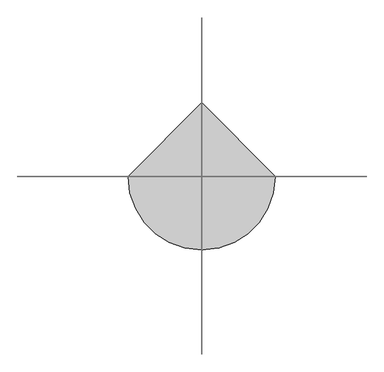
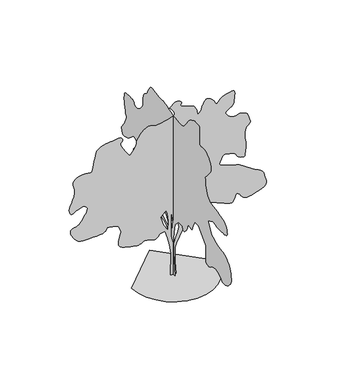
"""IFC4 building model written with IfcOpenShell, lengths in millimetres: proxy geometry, blueberry elder 26160 : blueberry elder 26160."""

from ifc_helpers import new_model, si_unit, origin, place, context, project, spatial, triangles, source, transform, mapped, element, save


def entourage_a2d70376(model_context):
    return source(origin(), model_context, "Body", "Tessellation", [
        triangles([(-0.0014919, 59.6430573, 0.0042007), (-0.0014919, -63.4980182, 0.0042007), (-0.0014919, -15.6099892, 574.662743), (-0.0014919, -1.9275415, 923.5625221), (-0.0014919, -22.4510529, 1121.9570257), (-0.0014919, -77.1804997, 1347.7149754), (-0.0014919, -227.6865383, 1498.2227943), (-0.0014919, -385.0338381, 1498.2227943), (-0.0014919, -419.2400351, 1402.4443382), (-0.0014919, -487.6499219, 1409.2870892), (-0.0014919, -562.9051031, 1498.2227943), (-0.0014919, -610.791715, 1593.9986343), (-0.0014919, -638.1577045, 1689.7744743), (-0.0014919, -713.4103786, 1662.4110283), (-0.0014919, -795.5032602, 1655.5682774), (-0.0014919, -870.7558617, 1826.5992622), (-0.0014919, -925.4852972, 1929.2153824), (-0.0014919, -1075.9931162, 1922.3751022), (-0.0014919, -1192.2921947, 1826.5992622), (-0.0014919, -1404.3696568, 1600.8387691), (-0.0014919, -1411.2099369, 1375.0808922), (-0.0014919, -1409.1144253, 1348.2534599), (-0.0014919, -1404.5093285, 1316.2824463), (-0.0014919, -1399.9017609, 1281.557967), (-0.0014919, -1397.8062492, 1246.4730446), (-0.0014919, -1400.7374657, 1213.4249891), (-0.0014919, -1411.2099369, 1184.8042797), (-0.0014919, -1431.7331028, 1163.0034302), (-0.0014919, -1457.4226685, 1147.2477785), (-0.0014919, -1482.2740585, 1135.79746), (-0.0014919, -1507.1254486, 1129.6151339), (-0.0014919, -1532.8150143, 1129.6557564), (-0.0014919, -1560.1810764, 1136.8769726), (-0.0014919, -1590.0565784, 1152.2338114), (-0.0014919, -1623.2873989, 1176.6863886), (-0.0014919, -1664.49375, 1202.6350954), (-0.0014919, -1715.0347057, 1221.7613262), (-0.0014919, -1770.8411831, 1233.9482277), (-0.0014919, -1827.8439537, 1239.0739323), (-0.0014919, -1881.9739346, 1237.0215866), (-0.0014919, -1929.1645134, 1227.6667797), (-0.0014919, -1965.3442818, 1210.8926582), (-0.0014919, -1995.2630951, 1185.7212296), (-0.0014919, -2027.0942917, 1154.4487198), (-0.0014919, -2061.9177475, 1121.8579039), (-0.0014919, -2100.8127571, 1092.7367889), (-0.0014919, -2144.8513481, 1071.8757803), (-0.0014919, -2195.1129604, 1064.0551094), (-0.0014919, -2252.6744179, 1074.0677977), (-0.0014919, -2311.551638, 1100.7352833), (-0.0014919, -2364.3279224, 1137.4535362), (-0.0014919, -2409.9209244, 1180.8748684), (-0.0014919, -2447.2590523, 1227.6464321), (-0.0014919, -2475.2625755, 1274.4181412), (-0.0014919, -2492.8519089, 1317.8368572), (-0.0014919, -2498.9556061, 1354.5577263), (-0.0014919, -2495.0465424, 1394.6871082), (-0.0014919, -2484.4370155, 1446.9019444), (-0.0014919, -2468.7981445, 1505.7005356), (-0.0014919, -2449.8115128, 1565.5759506), (-0.0014919, -2429.1486752, 1621.024165), (-0.0014919, -2408.4858376, 1666.538538), (-0.0014919, -2389.496735, 1696.6146091), (-0.0014919, -2367.4393604, 1721.5473896), (-0.0014919, -2337.0025555, 1752.8198994), (-0.0014919, -2299.0269665, 1786.7288761), (-0.0014919, -2254.3509144, 1819.5584129), (-0.0014919, -2203.8099586, 1847.6000153), (-0.0014919, -2148.2422749, 1867.1453339), (-0.0014919, -2088.4861839, 1874.4858742), (-0.0014919, -2026.3171589, 1879.471907), (-0.0014919, -1963.0710194, 1893.4344269), (-0.0014919, -1898.9284229, 1914.8745426), (-0.0014919, -1834.0668297, 1942.2988861), (-0.0014919, -1768.6668972, 1974.2114731), (-0.0014919, -1702.9062309, 2009.1161739), (-0.0014919, -1636.9678139, 2045.5143883), (-0.0014919, -1493.3027458, 2312.3213585), (-0.0014919, -1712.220488, 2414.9399494), (-0.0014919, -1741.6996479, 2406.2024014), (-0.0014919, -1772.1365982, 2397.8254417), (-0.0014919, -1804.4885479, 2390.1673336), (-0.0014919, -1839.7108166, 2383.5861946), (-0.0014919, -1878.7633747, 2378.4401424), (-0.0014919, -1922.603722, 2375.0899109), (-0.0014919, -1972.187178, 2373.8910015), (-0.0014919, -2028.8316856, 2373.6725555), (-0.0014919, -2090.261657, 2373.8122272), (-0.0014919, -2152.0522167, 2375.5064552), (-0.0014919, -2209.7738388, 2379.9564743), (-0.0014919, -2258.9965611, 2388.3511654), (-0.0014919, -2295.2982697, 2401.8945248), (-0.0014919, -2314.2440609, 2421.7802296), (-0.0014919, -2317.876252, 2453.1136368), (-0.0014919, -2312.2908371, 2496.5351143), (-0.0014919, -2299.1666382, 2546.5297371), (-0.0014919, -2280.1775356, 2597.6091774), (-0.0014919, -2257.0026421, 2644.26912), (-0.0014919, -2231.3130764, 2680.9974014), (-0.0014919, -2204.7853352, 2702.2574409), (-0.0014919, -2178.018655, 2712.9253944), (-0.0014919, -2148.9788578, 2722.1454712), (-0.0014919, -2115.3923904, 2730.9847572), (-0.0014919, -2074.9835197, 2740.5606262), (-0.0014919, -2025.478838, 2751.9398735), (-0.0014919, -1964.605228, 2766.1637146), (-0.0014919, -1890.091753, 2784.3501045), (-0.0014919, -1810.2315113, 2802.4350471), (-0.0014919, -1735.3979977, 2817.522789), (-0.0014919, -1666.4267715, 2832.4579239), (-0.0014919, -1604.1586246, 2850.1870743), (-0.0014919, -1549.4291164, 2873.5298355), (-0.0014919, -1503.0767132, 2905.3557999), (-0.0014919, -1465.9392998, 2948.5613022), (-0.0014919, -1437.478537, 3000.783696), (-0.0014919, -1415.8377068, 3057.3241402), (-0.0014919, -1399.8814133, 3117.4716316), (-0.0014919, -1388.4717899, 3180.4634262), (-0.0014919, -1380.4732956, 3245.6399712), (-0.0014919, -1374.7506798, 3312.238813), (-0.0014919, -1370.1634598, 3379.5489487), (-0.0014919, -1421.161655, 3432.3047401), (-0.0014919, -1470.3080738, 3484.9335045), (-0.0014919, -1515.7412018, 3537.3337944), (-0.0014919, -1555.6115879, 3589.3785828), (-0.0014919, -1588.0626595, 3640.9149719), (-0.0014919, -1611.2401691, 3691.8929649), (-0.0014919, -1623.2873989, 3742.1340843), (-0.0014919, -1619.2183159, 3797.684182), (-0.0014919, -1597.4378139, 3860.6506874), (-0.0014919, -1561.1766552, 3925.0397804), (-0.0014919, -1513.6685085, 3984.9076378), (-0.0014919, -1458.1415199, 4034.2345688), (-0.0014919, -1397.8265968, 4067.0258812), (-0.0014919, -1335.9572628, 4077.3383331), (-0.0014919, -1278.5939037, 4074.2649742), (-0.0014919, -1229.7292992, 4071.8773293), (-0.0014919, -1189.4804478, 4071.7755913), (-0.0014919, -1157.966601, 4075.509375), (-0.0014919, -1135.3097717, 4084.6280045), (-0.0014919, -1121.6268133, 4100.6808037), (-0.0014919, -1117.0395206, 4125.2426765), (-0.0014919, -1118.7743711, 4171.0390091), (-0.0014919, -1122.5437632, 4241.9559013), (-0.0014919, -1126.1936857, 4326.2838936), (-0.0014919, -1127.5704185, 4412.288237), (-0.0014919, -1124.5173346, 4488.2344734), (-0.0014919, -1114.885655, 4542.4125618), (-0.0014919, -1096.5163548, 4563.0627548), (-0.0014919, -1069.6304232, 4564.4597626), (-0.0014919, -1037.2377783, 4567.5331215), (-0.0014919, -1001.3780485, 4570.6067711), (-0.0014919, -964.0806158, 4572.0037788), (-0.0014919, -927.380167, 4570.0477936), (-0.0014919, -893.3136417, 4563.0627548), (-0.0014919, -863.9156542, 4549.3976006), (-0.0014919, -835.993376, 4533.1416161), (-0.0014919, -805.556571, 4518.3587975), (-0.0014919, -773.4433422, 4503.0678703), (-0.0014919, -740.4944086, 4485.3895889), (-0.0014919, -707.545475, 4463.4185463), (-0.0014919, -675.4347897, 4435.2246277), (-0.0014919, -644.9979847, 4398.877137), (-0.0014919, -614.4824055, 4355.0112099), (-0.0014919, -581.8128516, 4307.6911331), (-0.0014919, -547.3475862, 4260.1167114), (-0.0014919, -511.4446541, 4215.5397812), (-0.0014919, -474.4672963, 4177.1857269), (-0.0014919, -436.7711234, 4148.2805145), (-0.0014919, -398.7168328, 4132.075399), (-0.0014919, -359.7633602, 4126.0048393), (-0.0014919, -319.1360072, 4124.6078316), (-0.0014919, -276.8322849, 4126.6905533), (-0.0014919, -232.8521387, 4131.0338928), (-0.0014919, -187.1978941, 4136.4696075), (-0.0014919, -139.8680069, 4141.7780045), (-0.0014919, -90.8629858, 4145.7658424), (-0.0014919, -33.0220578, 4153.2081207), (-0.0014919, 35.9481419, 4167.7368851), (-0.0014919, 108.7479043, 4186.3296455), (-0.0014919, 178.0769938, 4205.989492), (-0.0014919, 236.6359921, 4223.7439316), (-0.0014919, 277.1243819, 4236.5963448), (-0.0014919, 292.2424816, 4241.523951), (-0.0014919, 300.5609782, 4244.1147812), (-0.0014919, 323.5962728, 4250.5411331), (-0.0014919, 358.4806623, 4258.7705727), (-0.0014919, 402.3388501, 4266.7462486), (-0.0014919, 452.3032422, 4272.4357269), (-0.0014919, 505.495962, 4273.8327347), (-0.0014919, 559.0493792, 4268.9051285), (-0.0014919, 618.0663437, 4267.9400711), (-0.0014919, 686.0596498, 4278.836499), (-0.0014919, 757.7613779, 4295.8293571), (-0.0014919, 827.9085497, 4313.1774261), (-0.0014919, 891.2359343, 4325.1409401), (-0.0014919, 942.4728504, 4325.9789703), (-0.0014919, 976.3615522, 4309.9517509), (-0.0014919, 999.7371603, 4282.3926773), (-0.0014919, 1022.6327831, 4252.7761711), (-0.0014919, 1044.5733044, 4221.6359207), (-0.0014919, 1065.0761953, 4189.4032951), (-0.0014919, 1083.6639416, 4156.5608231), (-0.0014919, 1099.8614994, 4123.6171944), (-0.0014919, 1113.1837967, 4091.0287766), (-0.0014919, 1129.0994677, 4063.2159393), (-0.0014919, 1151.7182178, 4042.0067688), (-0.0014919, 1178.5228317, 4023.896537), (-0.0014919, 1207.0064129, 4005.4308037), (-0.0014919, 1234.6492023, 3983.1295486), (-0.0014919, 1258.9419056, 3953.5130424), (-0.0014919, 1277.3720306, 3913.1524246), (-0.0014919, 1288.5608826, 3878.2275215), (-0.0014919, 1294.0066257, 3861.6157448), (-0.0014919, 1295.50261, 3854.8086021), (-0.0014919, 1294.8448013, 3849.3223091), (-0.0014919, 1293.8262589, 3836.6730812), (-0.0014919, 1294.245274, 3808.3265556), (-0.0014919, 1297.8953419, 3755.7995293), (-0.0014919, 1304.3392799, 3695.8046448), (-0.0014919, 1312.5765678, 3648.6365936), (-0.0014919, 1323.5645599, 3611.1208603), (-0.0014919, 1338.2635174, 3580.2090843), (-0.0014919, 1357.6310852, 3552.7770378), (-0.0014919, 1382.622147, 3525.6752037), (-0.0014919, 1414.1969639, 3495.8555122), (-0.0014919, 1450.0566936, 3466.1628479), (-0.0014919, 1486.6377457, 3441.8806091), (-0.0014919, 1522.9750626, 3423.3131378), (-0.0014919, 1558.118557, 3410.8670952), (-0.0014919, 1591.1081131, 3404.8979828), (-0.0014919, 1620.9860859, 3405.7363037), (-0.0014919, 1646.795121, 3413.7628487), (-0.0014919, 1665.9440975, 3429.5107246), (-0.0014919, 1679.3451691, 3450.9992386), (-0.0014919, 1691.3136246, 3474.7736595), (-0.0014919, 1706.1523991, 3497.354258), (-0.0014919, 1728.1716946, 3515.2613045), (-0.0014919, 1761.6793877, 3525.0403587), (-0.0014919, 1810.9833549, 3523.2114006), (-0.0014919, 1870.0002468, 3519.655513), (-0.0014919, 1927.9427856, 3522.4495285), (-0.0014919, 1982.0524189, 3525.3702805), (-0.0014919, 2029.5835293, 3522.1698944), (-0.0014919, 2067.7775642, 3506.6504929), (-0.0014919, 2093.8862904, 3472.5891998), (-0.0014919, 2105.1536259, 3413.7628487), (-0.0014919, 2107.5870529, 3355.0888138), (-0.0014919, 2108.7045719, 3318.9189285), (-0.0014919, 2108.0264156, 3295.0939293), (-0.0014919, 2105.0749969, 3273.4275192), (-0.0014919, 2099.3701126, 3243.7095657), (-0.0014919, 2090.4343208, 3195.8305115), (-0.0014919, 2077.7901798, 3119.5796425), (-0.0014919, 2061.2548519, 3041.6777115), (-0.0014919, 2043.5255562, 2988.8966309), (-0.0014919, 2028.4253151, 2951.2030014), (-0.0014919, 2019.7893597, 2918.5384254), (-0.0014919, 2021.4453632, 2880.844796), (-0.0014919, 2037.2212898, 2828.0637154), (-0.0014919, 2070.9474289, 2750.1617844), (-0.0014919, 2114.4501514, 2668.4752007), (-0.0014919, 2155.0774681, 2607.7440239), (-0.0014919, 2189.9618214, 2562.9383286), (-0.0014919, 2216.2279507, 2529.0063881), (-0.0014919, 2231.0082985, 2500.9418221), (-0.0014919, 2231.4273136, 2473.7181931), (-0.0014919, 2214.6124969, 2442.3032501), (-0.0014919, 2195.0062809, 2409.7735497), (-0.0014919, 2184.256937, 2383.1061367), (-0.0014919, 2175.300943, 2363.1416576), (-0.0014919, 2161.0794273, 2350.7159626), (-0.0014919, 2134.5339546, 2346.6672272), (-0.0014919, 2088.6004211, 2351.8336269), (-0.0014919, 2016.218066, 2367.0507214), (-0.0014919, 1937.2366951, 2396.3496597), (-0.0014919, 1873.5715405, 2438.0946407), (-0.0014919, 1821.2754593, 2484.6274109), (-0.0014919, 1776.3986927, 2528.2875366), (-0.0014919, 1734.9940979, 2561.4142937), (-0.0014919, 1693.1069744, 2576.3494286), (-0.0014919, 1646.795121, 2565.45271), (-0.0014919, 1602.1392712, 2539.6566101), (-0.0014919, 1566.8155552, 2514.9450371), (-0.0014919, 1539.2717422, 2491.129921), (-0.0014919, 1517.9509506, 2468.0336563), (-0.0014919, 1501.2961533, 2445.4757309), (-0.0014919, 1487.7527939, 2423.2762138), (-0.0014919, 1475.7666069, 2401.2569183), (-0.0014919, 1494.8139908, 2382.2881634), (-0.0014919, 1513.8006226, 2363.8605091), (-0.0014919, 1532.6702557, 2346.5072079), (-0.0014919, 1551.3570511, 2330.7719765), (-0.0014919, 1569.8076691, 2317.1879219), (-0.0014919, 1587.9584507, 2306.2990517), (-0.0014919, 1605.7486439, 2298.6383274), (-0.0014919, 1624.7173988, 2295.1686264), (-0.0014919, 1645.2405647, 2294.3304508), (-0.0014919, 1665.5250824, 2292.895364), (-0.0014919, 1683.7749859, 2287.6299877), (-0.0014919, 1698.1945999, 2275.3032692), (-0.0014919, 1706.9905746, 2252.6845917), (-0.0014919, 1708.3672348, 2216.5455185), (-0.0014919, 1703.8180939, 2176.2559719), (-0.0014919, 1696.2794552, 2141.3512711), (-0.0014919, 1686.106675, 2108.8417728), (-0.0014919, 1673.6606323, 2075.7328926), (-0.0014919, 1659.3020611, 2039.0323711), (-0.0014919, 1643.3838467, 1995.7533268), (-0.0014919, 1626.2718098, 1942.8984135), (-0.0014919, 1608.601086, 1883.4013184), (-0.0014919, 1592.1266556, 1823.7848991), (-0.0014919, 1578.8829872, 1766.4443584), (-0.0014919, 1570.9048405, 1713.7673412), (-0.0014919, 1570.2266842, 1668.1539917), (-0.0014919, 1578.8829872, 1631.9944256), (-0.0014919, 1598.9083637, 1607.6815201), (-0.0014919, 1624.6970512, 1591.4839622), (-0.0014919, 1649.4087696, 1577.8035473), (-0.0014919, 1673.2237404, 1566.2135571), (-0.0014919, 1696.320005, 1556.3023888), (-0.0014919, 1718.8777851, 1547.6460857), (-0.0014919, 1741.0774475, 1539.8279583), (-0.0014919, 1763.096743, 1532.4263752), (-0.0014919, 1786.3707584, 1542.3400143), (-0.0014919, 1808.5702755, 1550.1581417), (-0.0014919, 1828.6159996, 1553.787862), (-0.0014919, 1845.4283455, 1551.135989), (-0.0014919, 1857.9352856, 1540.1073017), (-0.0014919, 1865.0549091, 1518.6062885), (-0.0014919, 1865.7127178, 1484.5397633), (-0.0014919, 1859.7895329, 1448.2787498), (-0.0014919, 1848.4813568, 1420.635815), (-0.0014919, 1832.6850826, 1400.1710758), (-0.0014919, 1813.2973125, 1385.4517708), (-0.0014919, 1791.2171196, 1375.040197), (-0.0014919, 1767.3435768, 1367.5015583), (-0.0014919, 1742.570961, 1361.3978611), (-0.0014919, 1730.8234222, 1353.9581989), (-0.0014919, 1718.9565594, 1345.8607281), (-0.0014919, 1706.8509029, 1336.4474945), (-0.0014919, 1694.3845127, 1325.0580734), (-0.0014919, 1681.4406807, 1311.0372723), (-0.0014919, 1667.8974667, 1293.7246662), (-0.0014919, 1653.6378719, 1272.4623013), (-0.0014919, 1633.9909607, 1249.8053993), (-0.0014919, 1605.3701786, 1228.5837296), (-0.0014919, 1569.2691845, 1208.558353), (-0.0014919, 1527.1838173, 1189.4905489), (-0.0014919, 1480.6129681, 1171.1415962), (-0.0014919, 1431.0498596, 1153.270158), (-0.0014919, 1379.9907669, 1135.6399841), (-0.0014919, 1215.8024603, 1231.4158241), (-0.0014919, 1051.6141537, 1108.2739946), (-0.0014919, 1029.6533575, 1105.4215525), (-0.0014919, 1007.8727829, 1103.0492409), (-0.0014919, 986.4529421, 1101.6318855), (-0.0014919, 965.5690424, 1101.6522331), (-0.0014919, 945.4065376, 1103.5877254), (-0.0014919, 926.1380917, 1107.915877), (-0.0014919, 907.9491583, 1115.1167456), (-0.0014919, 891.075915, 1124.6493759), (-0.0014919, 875.1577005, 1135.2589754), (-0.0014919, 859.4808231, 1146.3486328), (-0.0014919, 843.3263586, 1157.3188934), (-0.0014919, 825.97313, 1167.5703753), (-0.0014919, 806.7071548, 1176.5060944), (-0.0014919, 784.8072561, 1183.5266687), (-0.0014919, 760.1565805, 1188.9927595), (-0.0014919, 733.3493505, 1193.7399988), (-0.0014919, 704.7489887, 1197.8877834), (-0.0014919, 674.710924, 1201.5581263), (-0.0014919, 643.59589, 1204.8677353), (-0.0014919, 611.7645481, 1207.9411669), (-0.0014919, 579.5725814, 1210.8926582), (-0.0014919, 367.4951194, 1149.3204718), (-0.0014919, 189.6253804, 1019.3383621), (-0.0014919, 93.8490136, 861.9928791), (-0.0014919, 45.9605758, 560.9797846), (-0.0013978, 66.484046, 1115.1167456), (-0.0013978, 169.1019057, 1334.0344151), (-0.0013978, 4.9135321, 1402.4443382), (-0.0014104, 312.7656838, 1190.3694197), (-0.0014104, 476.9539541, 1299.8282181), (-0.0014104, 606.9360274, 1306.6684982), (-0.0014104, 716.3948622, 1368.2381413), (-0.0014104, 710.4918795, 1371.410622), (-0.0014104, 704.3476324, 1376.0181896), (-0.0014104, 697.7284143, 1383.4984016), (-0.0014104, 690.3878014, 1395.2840195), (-0.0014104, 682.089616, 1412.8176876), (-0.0014104, 672.5976082, 1437.529406), (-0.0014104, 661.6654266, 1470.8567322), (-0.0014104, 652.9303493, 1503.7853909), (-0.0014104, 649.5801178, 1527.3819157), (-0.0014104, 650.7155136, 1543.1985374), (-0.0014104, 655.442478, 1552.7921379), (-0.0014104, 662.864336, 1557.7172733), (-0.0014104, 672.0769278, 1559.5332962), (-0.0014104, 682.1912086, 1559.7924374), (-0.0014104, 689.0314161, 1641.8852463), (-0.0014104, 606.9360274, 1696.6146091), (-0.0014104, 429.0673059, 1546.1094063), (-0.0014104, 305.9254764, 1402.4443382), (-0.0014104, 223.8310687, 1286.1453323), (-0.0014104, 141.7369426, 1101.4337872), (67.7022311, 0.0002671, 0.0), (-69.1215849, 0.0002671, 0.0), (-62.2805962, 0.0002309, 560.9772411), (-96.4865524, 0.0002173, 807.2583567), (-144.3744815, 0.0002037, 1012.4930677), (-205.9448967, 0.0001946, 1197.2045403), (-329.0852182, 0.0001946, 1183.5241253), (-349.6693906, 0.0001946, 1154.5020596), (-370.6116806, 0.0001992, 1127.2782852), (-392.2728221, 0.0001992, 1103.6436087), (-415.0109327, 0.0001992, 1085.3936325), (-439.1841302, 0.0002037, 1074.3243227), (-465.1505685, 0.0002037, 1072.2288111), (-493.2734885, 0.0001992, 1080.9054617), (-523.1921565, 0.0001992, 1093.9686905), (-554.1877936, 0.0001992, 1104.1617456), (-586.0800694, 0.0001992, 1111.9595255), (-618.6886168, 0.0001992, 1117.8447041), (-651.8381922, 0.0001992, 1122.2922523), (-685.3458853, 0.0001992, 1125.7822283), (-719.0339453, 0.0001992, 1128.7946898), (-746.9764984, 0.0001992, 1112.8383963), (-775.4575361, 0.0001992, 1097.8981018), (-805.0180864, 0.0001992, 1084.9948923), (-836.191547, 0.0001992, 1075.1422234), (-869.5188732, 0.0002037, 1069.3586374), (-905.5412384, 0.0002037, 1068.6601336), (-944.7918222, 0.0002037, 1074.0652542), (-995.5334925, 0.0001992, 1083.856953), (-1060.8724548, 0.0001992, 1096.2826481), (-1133.6334206, 0.0001992, 1112.2999117), (-1206.6330345, 0.0001992, 1132.8637728), (-1272.690921, 0.0001946, 1158.9318037), (-1324.6262684, 0.0001946, 1191.4615768), (-1355.2613171, 0.0001901, 1231.4107372), (-1365.1546085, 0.0001901, 1279.0206219), (-1362.3630638, 0.0001856, 1331.6544731), (-1350.9534405, 0.0001811, 1385.9672916), (-1334.997147, 0.0001811, 1438.6012882), (-1318.5632664, 0.0001765, 1486.2110275), (-1305.7185562, 0.0001765, 1525.4413364), (-1300.5318089, 0.000172, 1552.9470703), (-1302.9068092, 0.000172, 1576.4623501), (-1309.4676006, 0.000172, 1604.5243), (-1319.3812397, 0.0001675, 1634.9815979), (-1331.8069347, 0.0001675, 1665.6773987), (-1345.9089809, 0.000163, 1694.4582001), (-1360.8467319, 0.000163, 1719.1699184), (-1375.7869537, 0.000163, 1737.6586155), (-1395.4313942, 0.000163, 1750.9224861), (-1424.0546471, 0.0001584, 1761.6716846), (-1460.1531704, 0.0001584, 1770.328133), (-1502.2385376, 0.0001584, 1777.3079395), (-1548.8093868, 0.0001584, 1783.0331715), (-1598.3724953, 0.0001584, 1787.9200825), (-1649.431588, 0.0001584, 1792.3879784), (-1657.3716557, 0.0001584, 1766.1802757), (-1668.9591751, 0.000163, 1741.0495422), (-1687.8465397, 0.000163, 1718.0726017), (-1717.6865788, 0.000163, 1698.3265686), (-1762.1238373, 0.000163, 1682.8885574), (-1824.8111446, 0.0001675, 1672.8377174), (-1909.398278, 0.0001675, 1669.2462215), (-2003.1193016, 0.0001675, 1666.9119164), (-2090.3809811, 0.0001675, 1662.3043488), (-2170.5789928, 0.0001675, 1659.0150146), (-2243.1190418, 0.0001675, 1660.6304684), (-2307.4039261, 0.0001675, 1670.7422058), (-2362.8293221, 0.000163, 1692.9418682), (-2408.80326, 0.000163, 1730.8183353), (-2450.3908379, 0.0001584, 1780.5998898), (-2490.1799789, 0.0001584, 1834.2117336), (-2523.8680389, 0.0001539, 1888.783548), (-2547.1392929, 0.0001494, 1941.4378922), (-2555.6992355, 0.0001449, 1989.3067726), (-2545.2344673, 0.0001449, 2029.5149288), (-2511.4219963, 0.0001449, 2059.1923325), (-2467.3223625, 0.0001403, 2077.8410488), (-2428.3689262, 0.0001403, 2089.431039), (-2393.8453068, 0.0001403, 2097.7876511), (-2363.0298912, 0.0001403, 2106.7437904), (-2335.2067348, 0.0001403, 2120.1269852), (-2309.6568409, 0.0001358, 2141.7653446), (-2285.6615032, 0.0001358, 2175.4939545), (-2257.2616379, 0.0001313, 2219.9110107), (-2222.6364258, 0.0001313, 2269.4739738), (-2187.2922169, 0.0001267, 2321.7904026), (-2156.7360878, 0.0001222, 2374.464949), (-2136.4719177, 0.0001222, 2425.1076427), (-2132.0040218, 0.0001177, 2471.3203743), (-2148.8391861, 0.0001177, 2510.7107025), (-2179.7535782, 0.0001132, 2538.5136566), (-2213.5406147, 0.0001132, 2553.0322472), (-2249.7203831, 0.0001132, 2556.4866875), (-2287.8154415, 0.0001132, 2551.0765526), (-2327.3479122, 0.0001132, 2539.0342644), (-2367.8355572, 0.0001132, 2522.5573631), (-2408.80326, 0.0001177, 2503.8704224), (-2437.9625267, 0.0001177, 2487.9929031), (-2466.1666191, 0.0001177, 2473.6141296), (-2492.453096, 0.0001177, 2462.2247086), (-2515.8670738, 0.0001177, 2455.3233856), (-2535.4554131, 0.0001177, 2454.4065811), (-2550.2635208, 0.0001177, 2460.9672272), (-2559.3059921, 0.0001177, 2476.5046509), (-2566.1387146, 0.0001177, 2495.7526039), (-2573.6824402, 0.0001177, 2514.0433479), (-2580.1340813, 0.0001132, 2533.7688881), (-2583.7155487, 0.0001132, 2557.3247177), (-2582.6487534, 0.0001132, 2587.0935402), (-2575.1047371, 0.0001086, 2625.4984634), (-2559.3059921, 0.0001041, 2674.9015526), (-2538.1680382, 0.0001041, 2727.6064751), (-2516.667025, 9.96e-05, 2775.7904526), (-2496.1235115, 9.96e-05, 2821.5612053), (-2477.8534058, 9.51e-05, 2867.0781944), (-2463.1746506, 9.05e-05, 2914.5505875), (-2453.4005379, 9.05e-05, 2966.0619781), (-2449.8498825, 8.6e-05, 3023.7962448), (-2453.8603935, 8.15e-05, 3079.1681557), (-2463.4920731, 8.15e-05, 3124.1261673), (-2475.1608376, 7.7e-05, 3161.6674805), (-2485.2727203, 7.7e-05, 3194.7637161), (-2490.240731, 7.24e-05, 3226.4376549), (-2486.4688683, 7.24e-05, 3259.6609177), (-2470.3753738, 6.79e-05, 3297.4559944), (-2440.0783859, 6.79e-05, 3333.6511688), (-2398.8922371, 6.34e-05, 3360.8800301), (-2351.003009, 6.34e-05, 3380.2093735), (-2300.601725, 6.34e-05, 3392.7059944), (-2251.8769375, 6.34e-05, 3399.4625587), (-2209.0144375, 6.34e-05, 3401.5708603), (-2176.2051029, 6.34e-05, 3400.0721146), (-2148.061908, 6.34e-05, 3394.4587944), (-2117.7647747, 6.34e-05, 3386.2290642), (-2087.3483173, 6.34e-05, 3379.4219215), (-2058.8468594, 6.34e-05, 3378.1263611), (-2034.2926895, 6.34e-05, 3386.4069603), (-2015.7253635, 6.34e-05, 3408.3271339), (-2005.174118, 5.88e-05, 3447.9511688), (-1996.2586739, 5.43e-05, 3505.228196), (-1982.4359711, 5.43e-05, 3573.6559959), (-1965.5043011, 4.98e-05, 3647.5697983), (-1947.2543976, 4.53e-05, 3721.3568642), (-1929.4820812, 4.07e-05, 3789.4035828), (-1913.985498, 3.62e-05, 3846.0963432), (-1902.5555271, 3.17e-05, 3885.7968269), (-1882.1516853, 3.17e-05, 3914.5241432), (-1842.3625443, 3.17e-05, 3941.473661), (-1788.9284512, 2.72e-05, 3965.6797417), (-1727.5976017, 2.72e-05, 3986.1523293), (-1664.1128139, 2.72e-05, 4001.9763634), (-1604.2170513, 2.72e-05, 4012.1617882), (-1553.655748, 2.72e-05, 4015.7685448), (-1506.505719, 2.72e-05, 4019.2738541), (-1455.4059311, 2.72e-05, 4027.0969231), (-1403.9480255, 2.72e-05, 4035.1487572), (-1355.7210274, 2.26e-05, 4039.3906494), (-1314.3139618, 2.72e-05, 4035.7077347), (-1283.3207954, 2.72e-05, 4020.0865952), (-1266.3256119, 2.72e-05, 3988.4126564), (-1265.9090675, 3.17e-05, 3953.5130424), (-1277.2170982, 3.17e-05, 3927.1225021), (-1292.7136814, 3.17e-05, 3903.5003975), (-1304.8625038, 3.62e-05, 3876.8813828), (-1306.1173691, 3.62e-05, 3841.4989494), (-1288.9442894, 4.07e-05, 3791.6642006), (-1245.8049168, 4.53e-05, 3721.6109184), (-1194.5655298, 4.98e-05, 3646.731768), (-1155.891437, 4.98e-05, 3586.6860146), (-1126.4324793, 5.43e-05, 3542.0835045), (-1102.8384253, 5.43e-05, 3513.5340843), (-1081.7563545, 5.88e-05, 3501.5958595), (-1059.8361809, 5.43e-05, 3506.9045471), (-1033.7274548, 5.43e-05, 3530.0441231), (-1006.0846653, 5.43e-05, 3563.4705711), (-981.7894913, 4.98e-05, 3598.9288719), (-960.8472376, 4.98e-05, 3635.9620766), (-943.2576862, 4.53e-05, 3674.0620766), (-929.0158957, 4.53e-05, 3712.7463432), (-918.1268801, 4.07e-05, 3751.557637), (-910.5856253, 4.07e-05, 3790.0131386), (-896.7832701, 3.62e-05, 3834.3363052), (-868.8610645, 3.17e-05, 3887.3714401), (-829.4503887, 3.17e-05, 3943.65783), (-781.1826954, 2.72e-05, 3997.6838928), (-726.6920534, 2.26e-05, 4043.9118851), (-668.6123863, 2.26e-05, 4076.8558044), (-609.5750742, 2.26e-05, 4091.0287766), (-561.6655712, 2.26e-05, 4089.1745293), (-529.5548495, 2.26e-05, 4080.3608231), (-504.7415749, 2.26e-05, 4068.5752052), (-478.734514, 2.26e-05, 4057.7549355), (-443.0322238, 2.26e-05, 4051.836692), (-389.1410002, 2.26e-05, 4054.7577347), (-308.5619797, 2.26e-05, 4070.5056107), (-218.1912603, 2.26e-05, 4091.0034874), (-140.9838273, 2.26e-05, 4107.2086029), (-77.5383903, 1.81e-05, 4121.4836037), (-28.4536116, 1.81e-05, 4136.2408424), (5.6723577, 1.81e-05, 4153.8685455), (24.2412211, 1.81e-05, 4176.7540672), (26.6545277, 1.36e-05, 4207.310051), (18.5968788, 1.36e-05, 4240.5080246), (6.5899843, 9.1e-06, 4270.098951), (-8.707838, 9.1e-06, 4296.7182564), (-26.6385244, 9.1e-06, 4320.924337), (-46.5435071, 4.5e-06, 4343.3526192), (-67.764968, 4.5e-06, 4364.5617897), (-89.6448007, 4.5e-06, 4385.1864029), (-61.8612404, 4.5e-06, 4411.3740486), (-34.4965295, 0.0, 4436.3675812), (-7.9696625, 0.0, 4458.9734688), (17.3007665, 0.0, 4477.9728905), (40.8958095, 0.0, 4492.1967316), (62.3966728, -4.5e-06, 4500.4264618), (81.3844583, -4.5e-06, 4501.4932571), (101.1299282, -4.5e-06, 4497.6833153), (123.747879, 0.0, 4491.9682571), (147.0833914, 0.0, 4484.0687393), (168.9832901, 0.0, 4473.8071564), (187.292892, 0.0, 4460.9038742), (199.8582769, 0.0, 4445.1304184), (204.5255429, 0.0, 4426.2330254), (200.2771285, 4.5e-06, 4409.087851), (190.6436686, 4.5e-06, 4397.0737587), (180.2923927, 4.5e-06, 4387.8281021), (173.8900582, 4.5e-06, 4378.9382378), (176.103931, 4.5e-06, 4367.9906502), (191.6012409, 4.5e-06, 4352.6491447), (225.0492538, 9.1e-06, 4330.4749168), (270.045399, 9.1e-06, 4307.8943184), (316.1184952, 9.1e-06, 4291.4095688), (361.8334373, 9.1e-06, 4278.7603409), (405.7526316, 9.1e-06, 4267.6860168), (446.4409184, 1.36e-05, 4255.8751099), (482.4607038, 1.36e-05, 4241.0667114), (512.3793717, 1.36e-05, 4221.0007851), (536.1741039, 1.36e-05, 4195.1436424), (555.3003347, 1.81e-05, 4164.9937386), (570.5378131, 1.81e-05, 4131.2623672), (582.6637808, 2.26e-05, 4094.6355331), (592.4580231, 2.26e-05, 4055.8498192), (600.6952383, 2.72e-05, 4015.6415176), (608.1552117, 2.72e-05, 3974.722213), (703.9310881, 2.26e-05, 4063.647599), (703.2935543, 2.26e-05, 4067.2543556), (702.1759626, 2.26e-05, 4077.3127533), (701.7771498, 2.26e-05, 4092.7307076), (703.2935543, 2.26e-05, 4112.4920013), (707.9213968, 1.81e-05, 4135.4533905), (716.8571886, 1.81e-05, 4160.59953), (731.2970776, 1.81e-05, 4186.7868851), (747.8502823, 1.36e-05, 4214.0666153), (763.2096645, 1.36e-05, 4241.5748199), (778.6859001, 9.1e-06, 4267.025592), (795.599766, 9.1e-06, 4288.2091827), (815.2644814, 9.1e-06, 4302.7888161), (838.9982071, 9.1e-06, 4308.5038742), (868.119322, 9.1e-06, 4303.0937393), (898.3758327, 9.1e-06, 4289.9872719), (925.0433184, 9.1e-06, 4274.3408432), (948.7186901, 1.36e-05, 4256.6116928), (969.9988592, 1.36e-05, 4237.2059006), (989.4857512, 1.36e-05, 4216.5304184), (1007.7737337, 1.36e-05, 4195.0419044), (1025.4674212, 1.81e-05, 4173.1217308), (1029.993671, 1.81e-05, 4151.4047424), (1035.2997425, 1.81e-05, 4131.2879471), (1042.1602976, 1.81e-05, 4114.4224068), (1051.3550852, 2.26e-05, 4102.3827347), (1063.6613834, 2.26e-05, 4096.8199928), (1079.8564705, 2.26e-05, 4099.3346649), (1100.7200226, 2.26e-05, 4111.5522331), (1123.5978413, 1.81e-05, 4132.811982), (1146.3537197, 1.81e-05, 4159.3295494), (1170.5472284, 1.81e-05, 4188.0062874), (1197.732851, 1.36e-05, 4215.7429665), (1229.4650711, 1.36e-05, 4239.3903603), (1267.3009884, 1.36e-05, 4255.8751099), (1312.7950138, 1.36e-05, 4262.0471169), (1361.8805351, 9.1e-06, 4267.2796463), (1408.0932667, 9.1e-06, 4278.7350517), (1449.398885, 9.1e-06, 4290.06343), (1483.7651012, 9.1e-06, 4294.9148781), (1509.1549759, 9.1e-06, 4286.9900711), (1523.5363655, 1.36e-05, 4259.888237), (1524.8724758, 1.36e-05, 4207.310051), (1519.9652172, 1.81e-05, 4142.8703796), (1515.7766647, 2.26e-05, 4084.5009773), (1510.5112885, 2.72e-05, 4032.4817688), (1502.3755932, 2.72e-05, 3987.0412285), (1489.5689621, 3.17e-05, 3948.43312), (1470.3029869, 3.17e-05, 3916.8862083), (1442.7795216, 3.17e-05, 3892.6292587), (1408.3320602, 3.62e-05, 3872.7156487), (1372.4519829, 3.62e-05, 3853.18312), (1339.5615486, 3.62e-05, 3832.6852432), (1314.0928997, 3.62e-05, 3809.9014595), (1300.4709114, 4.07e-05, 3783.5362083), (1303.1226391, 4.07e-05, 3752.243351), (1326.4778996, 4.53e-05, 3714.7529068), (1361.2023788, 4.53e-05, 3678.8882355), (1394.8497437, 4.98e-05, 3652.3703773), (1427.1814911, 4.98e-05, 3633.6253006), (1457.9560661, 4.98e-05, 3621.1030998), (1486.937582, 4.98e-05, 3613.2291618), (1513.8818676, 4.98e-05, 3608.4791611), (1538.5553616, 4.98e-05, 3605.3043549), (1559.4774857, 4.98e-05, 3606.8028099), (1576.9297634, 4.98e-05, 3614.7531967), (1593.3026012, 4.98e-05, 3625.5734665), (1610.9962887, 4.98e-05, 3635.7080223), (1632.3958546, 4.98e-05, 3641.4992386), (1659.9014431, 4.98e-05, 3639.4165169), (1695.9009899, 4.98e-05, 3625.8275208), (1734.0771481, 4.98e-05, 3609.6729836), (1766.7466656, 4.98e-05, 3599.6145859), (1794.2701309, 4.98e-05, 3591.7153587), (1817.0082779, 4.98e-05, 3582.0124626), (1835.316608, 5.43e-05, 3566.5945084), (1849.558326, 5.43e-05, 3541.4486595), (1860.0892239, 5.88e-05, 3502.6882347), (1872.6545906, 5.88e-05, 3459.6350487), (1889.4085098, 6.34e-05, 3423.0590836), (1905.3241081, 6.34e-05, 3391.0296432), (1915.3774189, 6.34e-05, 3361.6419022), (1914.5392433, 6.79e-05, 3332.939875), (1897.7853241, 6.79e-05, 3303.0693146), (1860.0892239, 7.24e-05, 3270.0748169), (1819.3424377, 7.24e-05, 3225.0150673), (1794.6308647, 7.7e-05, 3164.2835999), (1782.7233067, 8.15e-05, 3093.9765541), (1780.3890015, 8.6e-05, 3020.2147774), (1784.397187, 9.05e-05, 2949.0694107), (1791.5192814, 9.51e-05, 2886.6615921), (1798.5195808, 9.51e-05, 2839.0871704), (1802.5886639, 9.96e-05, 2800.3776146), (1803.4268394, 9.96e-05, 2760.5756836), (1801.5701214, 0.0001041, 2719.8848534), (1797.5619358, 0.0001041, 2678.48302), (1791.9384418, 0.0001086, 2636.5474983), (1785.2353626, 0.0001086, 2594.2311859), (1777.9964149, 0.0001132, 2551.7622665), (1779.0935863, 0.0001132, 2530.0377205), (1777.9760674, 0.0001177, 2509.9334244), (1772.4312023, 0.0001177, 2493.0603264), (1760.2443008, 0.0001177, 2481.0334442), (1739.2028526, 0.0001177, 2475.4680862), (1707.0896965, 0.0001177, 2477.9801422), (1661.6947929, 0.0001177, 2490.1875366), (1618.3547058, 0.0001177, 2511.8867935), (1589.7339237, 0.0001132, 2539.8115425), (1569.6094254, 0.0001132, 2570.9645828), (1551.7583347, 0.0001086, 2602.3591782), (1529.9574852, 0.0001086, 2631.0103363), (1497.9864716, 0.0001086, 2653.895858), (1449.6198017, 0.0001086, 2668.0688301), (1395.7870411, 0.0001041, 2678.0257805), (1350.6918285, 0.0001041, 2688.3635216), (1313.0159306, 0.0001041, 2696.0598541), (1281.4411137, 0.0001041, 2698.1425758), (1254.6568474, 0.0001041, 2691.5894875), (1231.339666, 0.0001041, 2673.4536758), (1210.1788937, 0.0001086, 2640.6876526), (1189.6938068, 0.0001086, 2600.6063782), (1171.1263355, 0.0001132, 2562.9127487), (1157.2249311, 0.0001132, 2528.3229996), (1150.7428413, 0.0001177, 2497.566156), (1154.4309156, 0.0001177, 2471.3584534), (1171.0450905, 0.0001177, 2450.416127), (1203.3361427, 0.0001222, 2435.4580284), (1238.8200233, 0.0001222, 2424.8078064), (1266.0436523, 0.0001222, 2415.5926712), (1289.3202839, 0.0001222, 2406.7382698), (1312.9550331, 0.0001222, 2397.1625462), (1341.2582474, 0.0001222, 2385.7959435), (1378.5353325, 0.0001222, 2371.5542255), (1429.0966358, 0.0001267, 2353.3652195), (1483.0867996, 0.0001267, 2336.5300552), (1529.2996765, 0.0001267, 2325.0823528), (1570.0082382, 0.0001267, 2316.0272369), (1607.4860378, 0.0001267, 2306.3725937), (1644.0035763, 0.0001267, 2293.1290707), (1681.8394936, 0.0001313, 2273.3044086), (1723.2669067, 0.0001313, 2243.9063484), (1969.5480949, 0.0001403, 2072.8753635), (2012.7713287, 0.0001449, 2045.9309326), (2063.1724674, 0.0001449, 2021.4962322), (2116.2052769, 0.0001449, 1996.2256817), (2167.325267, 0.0001494, 1966.766724), (2211.9811169, 0.0001494, 1929.7691277), (2245.6284817, 0.0001539, 1881.8823704), (2263.7183659, 0.0001584, 1819.7514244), (2277.1220535, 0.000163, 1754.133046), (2294.714003, 0.000163, 1696.8914818), (2308.9558662, 0.0001675, 1646.350526), (2312.3060978, 0.000172, 1600.8336823), (2297.226059, 0.000172, 1558.6696861), (2256.1797272, 0.0001765, 1518.1820412), (2181.6255569, 0.0001765, 1477.6943962), (2092.3901608, 0.0001811, 1441.2352844), (2012.2505756, 0.0001811, 1413.8692223), (1941.0873322, 0.0001811, 1395.4796471), (1878.7784901, 0.0001811, 1385.9470894), (1825.2048706, 0.0001811, 1385.1494637), (1780.2493298, 0.0001811, 1392.9675911), (1743.7900726, 0.0001811, 1409.2820023), (1711.9766075, 0.0001811, 1437.6234409), (1681.1232582, 0.0001765, 1476.018045), (1651.3442619, 0.0001765, 1516.0891457), (1622.764175, 0.000172, 1549.4571671), (1595.4972347, 0.000172, 1567.7451496), (1569.667852, 0.000172, 1562.581366), (1545.3956417, 0.0001765, 1525.5811535), (1524.8724758, 0.0001765, 1474.8801785), (1508.5377171, 0.0001811, 1434.1130447), (1493.8768387, 0.0001811, 1403.1581028), (1478.3802555, 0.0001811, 1381.8982086), (1459.5334408, 0.0001856, 1370.2092419), (1434.8192516, 0.0001856, 1367.9765293), (1401.7305737, 0.0001856, 1375.0758053), (1362.2209213, 0.0001811, 1387.9992897), (1320.1965969, 0.0001811, 1403.0793285), (1276.0767609, 0.0001811, 1419.9525719), (1230.2830444, 0.0001811, 1438.260902), (1183.231992, 0.0001765, 1457.6488174), (1135.34538, 0.0001765, 1477.7528229), (1087.0370642, 0.0001765, 1498.2177074), (758.6605236, 0.0001675, 1635.0398792), (567.1088073, 0.000172, 1552.9470703), (423.4437392, 0.0001856, 1361.3927742), (245.5724742, 0.0001992, 1101.4287003), (74.5432198, 0.0002173, 800.4181492), (47.1785065, 0.0002218, 697.7994856), (47.1785065, 0.0002309, 567.8174486), (47.1785065, 0.000249, 294.1703436), (-0.7096842, 8.15e-05, 773.0521597), (67.7022311, 6.79e-05, 964.6063831), (122.4313987, 5.88e-05, 1087.7457418), (142.9546191, 5.43e-05, 1197.2045403), (122.4313987, 4.53e-05, 1320.3464424), (60.8604794, 4.53e-05, 1347.7123592), (50.6288455, 4.53e-05, 1339.2134594), (40.5767883, 4.53e-05, 1332.5129963), (30.8833756, 4.53e-05, 1329.4015583), (21.7287019, 4.53e-05, 1331.6748207), (13.2919576, 4.53e-05, 1341.1287495), (5.7526473, 4.53e-05, 1359.5590199), (-0.7096842, 4.07e-05, 1388.7588364), (-6.9725849, 4.07e-05, 1423.9404099), (-13.9534758, 4.07e-05, 1459.1244541), (-21.5326905, 3.62e-05, 1494.3086437), (-29.5905153, 3.62e-05, 1529.4902172), (-38.0073208, 3.17e-05, 1564.6742615), (-46.6636488, 3.17e-05, 1599.8584511), (-55.4393531, 2.72e-05, 1635.0398792), (-62.2805962, 4.98e-05, 1299.8231312), (-55.4393531, 6.34e-05, 1019.3358187), (-130.6925041, 8.6e-05, 1204.0472912), (-123.8507524, 7.24e-05, 1443.4881992), (-144.3744815, 6.34e-05, 1635.0398792), (-178.5804332, 5.43e-05, 1744.4987503), (-246.9923367, 5.88e-05, 1676.0863564), (-315.4047669, 6.34e-05, 1600.8336823), (-240.1508393, 7.7e-05, 1375.0758053), (-1032.8410263, 0.0, 0.0044904), (-1005.5360069, -236.6588468, 0.0044904), (-927.7712769, -453.992347, 0.0044904), (-805.775017, -645.7726467, 0.0044904), (-645.7726467, -805.775017, 0.0044904), (-453.992347, -927.7712769, 0.0044904), (-236.6588468, -1005.5360069, 0.0044904), (4.51e-05, -1032.8410263, 0.0044904), (236.6588468, -1005.5360069, 0.0044904), (453.992347, -927.7712769, 0.0044904), (645.7726467, -805.775017, 0.0044904), (805.775017, -645.7726467, 0.0044904), (927.7712769, -453.992347, 0.0044904), (1005.5360069, -236.6588468, 0.0044904), (1032.8410263, 9.05e-05, 0.0044904), (-0.0001354, 1032.8410263, 0.0044904)], [[379, 1, 382], [380, 404, 405], [379, 382, 380], [378, 379, 380], [404, 380, 381], [380, 405, 406], [377, 378, 380], [377, 380, 406], [376, 377, 406], [376, 406, 383], [376, 383, 384], [375, 376, 384], [375, 384, 385], [374, 375, 385], [1, 2, 3], [373, 374, 385], [373, 385, 386], [372, 373, 386], [371, 372, 386], [370, 371, 386], [8, 9, 10], [8, 10, 11], [369, 370, 386], [14, 15, 16], [13, 14, 16], [368, 369, 386], [8, 11, 12], [367, 368, 386], [8, 12, 13], [351, 352, 353], [404, 381, 382], [403, 404, 382], [148, 149, 150], [147, 148, 150], [147, 150, 151], [146, 147, 151], [146, 151, 152], [146, 152, 153], [146, 153, 154], [145, 146, 154], [145, 154, 155], [145, 155, 156], [145, 156, 157], [145, 157, 158], [144, 145, 158], [144, 158, 159], [144, 159, 160], [144, 160, 161], [144, 161, 162], [144, 162, 163], [143, 144, 163], [143, 163, 164], [143, 164, 165], [142, 143, 165], [142, 165, 166], [141, 142, 166], [141, 166, 167], [141, 167, 168], [141, 168, 169], [140, 141, 169], [366, 367, 386], [350, 351, 353], [7, 8, 13], [92, 93, 94], [91, 92, 94], [91, 94, 95], [90, 91, 95], [90, 95, 96], [89, 90, 96], [89, 96, 97], [88, 89, 97], [88, 97, 98], [88, 98, 99], [88, 99, 100], [88, 100, 101], [88, 101, 102], [88, 102, 103], [87, 88, 103], [87, 103, 104], [87, 104, 105], [86, 87, 105], [86, 105, 106], [85, 86, 106], [84, 85, 106], [84, 106, 107], [83, 84, 107], [82, 83, 107], [81, 82, 107], [81, 107, 108], [80, 81, 108], [79, 80, 108], [79, 108, 109], [79, 109, 110], [78, 79, 110], [78, 110, 111], [78, 111, 112], [78, 112, 113], [78, 113, 114], [349, 350, 353], [271, 272, 273], [270, 271, 273], [270, 273, 274], [269, 270, 274], [269, 274, 275], [268, 269, 275], [268, 275, 276], [267, 268, 276], [266, 267, 276], [265, 266, 276], [264, 265, 276], [263, 264, 276], [262, 263, 276], [262, 276, 277], [262, 277, 278], [261, 262, 278], [261, 278, 279], [260, 261, 279], [260, 279, 280], [259, 260, 280], [259, 280, 281], [258, 259, 281], [258, 281, 282], [327, 328, 329], [327, 329, 330], [326, 327, 330], [326, 330, 331], [325, 326, 331], [325, 331, 332], [324, 325, 332], [324, 332, 333], [324, 333, 334], [324, 334, 335], [324, 335, 336], [324, 336, 337], [324, 337, 338], [323, 324, 338], [322, 323, 338], [322, 338, 339], [321, 322, 339], [321, 339, 340], [320, 321, 340], [320, 340, 341], [320, 341, 342], [319, 320, 342], [319, 342, 343], [318, 319, 343], [318, 343, 344], [317, 318, 344], [317, 344, 345], [317, 345, 346], [317, 346, 347], [317, 347, 348], [317, 348, 349], [317, 349, 353], [316, 317, 353], [315, 316, 353], [314, 315, 353], [257, 258, 282], [13, 16, 17], [365, 366, 386], [244, 245, 246], [244, 246, 247], [243, 244, 247], [243, 247, 248], [242, 243, 248], [241, 242, 248], [241, 248, 249], [241, 249, 250], [241, 250, 251], [241, 251, 252], [241, 252, 253], [240, 241, 253], [240, 253, 254], [239, 240, 254], [238, 239, 254], [237, 238, 254], [236, 237, 254], [235, 236, 254], [234, 235, 254], [233, 234, 254], [233, 254, 255], [233, 255, 256], [233, 256, 257], [233, 257, 282], [232, 233, 282], [231, 232, 282], [230, 231, 282], [230, 282, 283], [229, 230, 283], [229, 283, 284], [228, 229, 284], [228, 284, 285], [227, 228, 285], [227, 285, 286], [226, 227, 286], [226, 286, 287], [225, 226, 287], [225, 287, 288], [224, 225, 288], [224, 288, 289], [396, 397, 398], [396, 398, 399], [395, 396, 399], [395, 399, 400], [394, 395, 400], [393, 394, 400], [392, 393, 400], [353, 354, 355], [223, 224, 289], [140, 169, 170], [300, 301, 302], [299, 300, 302], [299, 302, 303], [298, 299, 303], [297, 298, 303], [297, 303, 304], [296, 297, 304], [296, 304, 305], [296, 305, 306], [295, 296, 306], [295, 306, 307], [295, 307, 308], [294, 295, 308], [294, 308, 309], [293, 294, 309], [292, 293, 309], [292, 309, 310], [291, 292, 310], [291, 310, 311], [290, 291, 311], [289, 290, 311], [289, 311, 312], [353, 355, 356], [353, 356, 357], [353, 357, 358], [353, 358, 359], [353, 359, 360], [353, 360, 361], [353, 361, 362], [353, 362, 363], [353, 363, 364], [353, 364, 365], [353, 365, 386], [314, 353, 386], [313, 314, 386], [313, 386, 387], [313, 387, 388], [313, 388, 389], [313, 389, 390], [313, 390, 391], [313, 391, 392], [313, 392, 400], [313, 400, 401], [312, 313, 401], [289, 312, 401], [289, 401, 402], [223, 289, 402], [222, 223, 402], [221, 222, 402], [221, 402, 403], [221, 403, 382], [220, 221, 382], [219, 220, 382], [218, 219, 382], [217, 218, 382], [196, 197, 198], [196, 198, 199], [195, 196, 199], [195, 199, 200], [195, 200, 201], [194, 195, 201], [194, 201, 202], [194, 202, 203], [194, 203, 204], [194, 204, 205], [193, 194, 205], [193, 205, 206], [192, 193, 206], [78, 114, 115], [216, 217, 382], [26, 27, 28], [26, 28, 29], [25, 26, 29], [24, 25, 29], [24, 29, 30], [24, 30, 31], [24, 31, 32], [24, 32, 33], [24, 33, 34], [24, 34, 35], [23, 24, 35], [22, 23, 35], [22, 35, 36], [21, 22, 36], [21, 36, 37], [20, 21, 37], [20, 37, 38], [20, 38, 39], [20, 39, 40], [20, 40, 41], [192, 206, 207], [191, 192, 207], [215, 216, 382], [214, 215, 382], [213, 214, 382], [212, 213, 382], [211, 212, 382], [210, 211, 382], [209, 210, 382], [208, 209, 382], [207, 208, 382], [191, 207, 382], [190, 191, 382], [189, 190, 382], [188, 189, 382], [187, 188, 382], [186, 187, 382], [185, 186, 382], [184, 185, 382], [183, 184, 382], [182, 183, 382], [181, 182, 382], [180, 181, 382], [179, 180, 382], [178, 179, 382], [177, 178, 382], [176, 177, 382], [175, 176, 382], [174, 175, 382], [173, 174, 382], [172, 173, 382], [171, 172, 382], [170, 171, 382], [140, 170, 382], [139, 140, 382], [138, 139, 382], [137, 138, 382], [136, 137, 382], [135, 136, 382], [134, 135, 382], [133, 134, 382], [132, 133, 382], [131, 132, 382], [130, 131, 382], [129, 130, 382], [47, 48, 49], [46, 47, 49], [46, 49, 50], [45, 46, 50], [45, 50, 51], [44, 45, 51], [44, 51, 52], [43, 44, 52], [43, 52, 53], [43, 53, 54], [43, 54, 55], [43, 55, 56], [43, 56, 57], [43, 57, 58], [43, 58, 59], [42, 43, 59], [42, 59, 60], [42, 60, 61], [42, 61, 62], [42, 62, 63], [42, 63, 64], [42, 64, 65], [42, 65, 66], [41, 42, 66], [20, 41, 66], [20, 66, 67], [20, 67, 68], [20, 68, 69], [20, 69, 70], [20, 70, 71], [20, 71, 72], [20, 72, 73], [20, 73, 74], [20, 74, 75], [20, 75, 76], [19, 20, 76], [19, 76, 77], [19, 77, 78], [18, 19, 78], [18, 78, 115], [17, 18, 115], [17, 115, 116], [17, 116, 117], [17, 117, 118], [13, 17, 118], [7, 13, 118], [7, 118, 119], [7, 119, 120], [7, 120, 121], [127, 128, 129], [126, 127, 129], [125, 126, 129], [124, 125, 129], [123, 124, 129], [122, 123, 129], [121, 122, 129], [121, 129, 382], [7, 121, 382], [6, 7, 382], [5, 6, 382], [4, 5, 382], [4, 382, 1], [4, 1, 3], [843, 407, 844], [842, 843, 844], [863, 866, 867], [866, 863, 864], [841, 842, 844], [863, 867, 868], [866, 864, 865], [840, 841, 844], [840, 844, 845], [839, 840, 845], [839, 845, 846], [839, 846, 847], [838, 839, 847], [838, 847, 848], [844, 407, 408], [844, 408, 409], [844, 409, 410], [865, 844, 410], [865, 410, 411], [866, 865, 411], [866, 411, 412], [872, 866, 412], [872, 412, 413], [615, 616, 617], [863, 868, 869], [614, 615, 617], [614, 617, 618], [613, 614, 618], [613, 618, 619], [837, 838, 848], [837, 848, 849], [613, 619, 620], [612, 613, 620], [612, 620, 621], [612, 621, 622], [612, 622, 623], [612, 623, 624], [612, 624, 625], [612, 625, 626], [612, 626, 627], [612, 627, 628], [612, 628, 629], [612, 629, 630], [612, 630, 631], [612, 631, 632], [612, 632, 633], [612, 633, 634], [612, 634, 635], [611, 612, 635], [610, 611, 635], [610, 635, 636], [609, 610, 636], [609, 636, 637], [609, 637, 638], [608, 609, 638], [608, 638, 639], [691, 692, 693], [690, 691, 693], [690, 693, 694], [689, 690, 694], [689, 694, 695], [688, 689, 695], [688, 695, 696], [687, 688, 696], [687, 696, 697], [686, 687, 697], [685, 686, 697], [684, 685, 697], [683, 684, 697], [683, 697, 698], [682, 683, 698], [682, 698, 699], [682, 699, 700], [682, 700, 701], [682, 701, 702], [682, 702, 703], [681, 682, 703], [681, 703, 704], [680, 681, 704], [680, 704, 705], [679, 680, 705], [679, 705, 706], [678, 679, 706], [871, 872, 413], [608, 639, 640], [509, 510, 511], [508, 509, 511], [508, 511, 512], [507, 508, 512], [506, 507, 512], [506, 512, 513], [506, 513, 514], [505, 506, 514], [505, 514, 515], [505, 515, 516], [505, 516, 517], [504, 505, 517], [504, 517, 518], [503, 504, 518], [503, 518, 519], [502, 503, 519], [502, 519, 520], [501, 502, 520], [501, 520, 521], [500, 501, 521], [500, 521, 522], [500, 522, 523], [499, 500, 523], [499, 523, 524], [498, 499, 524], [498, 524, 525], [565, 566, 567], [565, 567, 568], [564, 565, 568], [564, 568, 569], [564, 569, 570], [563, 564, 570], [563, 570, 571], [562, 563, 571], [561, 562, 571], [561, 571, 572], [560, 561, 572], [559, 560, 572], [559, 572, 573], [558, 559, 573], [557, 558, 573], [556, 557, 573], [555, 556, 573], [554, 555, 573], [553, 554, 573], [552, 553, 573], [551, 552, 573], [550, 551, 573], [549, 550, 573], [549, 573, 574], [548, 549, 574], [547, 548, 574], [547, 574, 575], [546, 547, 575], [546, 575, 576], [546, 576, 577], [545, 546, 577], [545, 577, 578], [544, 545, 578], [544, 578, 579], [852, 853, 854], [851, 852, 854], [850, 851, 854], [850, 854, 855], [849, 850, 855], [849, 855, 856], [837, 849, 856], [837, 856, 857], [837, 857, 858], [837, 858, 859], [837, 859, 860], [837, 860, 861], [837, 861, 862], [837, 862, 863], [607, 608, 640], [481, 482, 483], [480, 481, 483], [480, 483, 484], [479, 480, 484], [479, 484, 485], [478, 479, 485], [478, 485, 486], [477, 478, 486], [477, 486, 487], [476, 477, 487], [475, 476, 487], [474, 475, 487], [473, 474, 487], [473, 487, 488], [472, 473, 488], [471, 472, 488], [471, 488, 489], [470, 471, 489], [470, 489, 490], [469, 470, 490], [469, 490, 491], [469, 491, 492], [468, 469, 492], [468, 492, 493], [467, 468, 493], [466, 467, 493], [465, 466, 493], [464, 465, 493], [463, 464, 493], [462, 463, 493], [462, 493, 494], [462, 494, 495], [461, 462, 495], [461, 495, 496], [460, 461, 496], [459, 460, 496], [458, 459, 496], [837, 863, 869], [836, 837, 869], [607, 640, 641], [871, 413, 414], [871, 414, 415], [871, 415, 416], [871, 416, 417], [871, 417, 418], [871, 418, 419], [871, 419, 420], [871, 420, 421], [871, 421, 422], [871, 422, 423], [871, 423, 424], [871, 424, 425], [871, 425, 426], [871, 426, 427], [457, 458, 496], [678, 706, 707], [607, 641, 642], [607, 642, 643], [607, 643, 644], [607, 644, 645], [607, 645, 646], [607, 646, 647], [607, 647, 648], [607, 648, 649], [607, 649, 650], [607, 650, 651], [606, 607, 651], [605, 606, 651], [677, 678, 707], [753, 754, 755], [752, 753, 755], [752, 755, 756], [751, 752, 756], [750, 751, 756], [750, 756, 757], [750, 757, 758], [749, 750, 758], [749, 758, 759], [749, 759, 760], [748, 749, 760], [748, 760, 761], [747, 748, 761], [747, 761, 762], [746, 747, 762], [745, 746, 762], [744, 745, 762], [744, 762, 763], [743, 744, 763], [742, 743, 763], [741, 742, 763], [741, 763, 764], [740, 741, 764], [740, 764, 765], [740, 765, 766], [739, 740, 766], [739, 766, 767], [739, 767, 768], [738, 739, 768], [738, 768, 769], [733, 734, 735], [732, 733, 735], [732, 735, 736], [731, 732, 736], [730, 731, 736], [730, 736, 737], [729, 730, 737], [672, 673, 674], [737, 738, 769], [729, 737, 769], [728, 729, 769], [727, 728, 769], [726, 727, 769], [725, 726, 769], [724, 725, 769], [723, 724, 769], [722, 723, 769], [721, 722, 769], [720, 721, 769], [719, 720, 769], [718, 719, 769], [717, 718, 769], [716, 717, 769], [715, 716, 769], [714, 715, 769], [713, 714, 769], [712, 713, 769], [711, 712, 769], [710, 711, 769], [709, 710, 769], [708, 709, 769], [708, 769, 770], [707, 708, 770], [677, 707, 770], [677, 770, 771], [677, 771, 772], [676, 677, 772], [676, 772, 773], [676, 773, 774], [825, 826, 827], [824, 825, 827], [824, 827, 828], [823, 824, 828], [823, 828, 829], [822, 823, 829], [822, 829, 830], [821, 822, 830], [821, 830, 831], [821, 831, 832], [820, 821, 832], [820, 832, 833], [820, 833, 834], [820, 834, 835], [820, 835, 836], [440, 441, 442], [439, 440, 442], [439, 442, 443], [438, 439, 443], [438, 443, 444], [438, 444, 445], [437, 438, 445], [437, 445, 446], [436, 437, 446], [436, 446, 447], [435, 436, 447], [435, 447, 448], [434, 435, 448], [433, 434, 448], [432, 433, 448], [431, 432, 448], [430, 431, 448], [429, 430, 448], [428, 429, 448], [427, 428, 448], [871, 427, 448], [871, 448, 449], [871, 449, 450], [871, 450, 451], [871, 451, 452], [871, 452, 453], [871, 453, 454], [870, 871, 454], [870, 454, 455], [869, 870, 455], [869, 455, 456], [804, 805, 806], [803, 804, 806], [803, 806, 807], [802, 803, 807], [801, 802, 807], [801, 807, 808], [800, 801, 808], [800, 808, 809], [799, 800, 809], [798, 799, 809], [797, 798, 809], [796, 797, 809], [795, 796, 809], [795, 809, 810], [794, 795, 810], [794, 810, 811], [794, 811, 812], [794, 812, 813], [794, 813, 814], [794, 814, 815], [794, 815, 816], [794, 816, 817], [794, 817, 818], [793, 794, 818], [793, 818, 819], [792, 793, 819], [792, 819, 820], [792, 820, 836], [791, 792, 836], [790, 791, 836], [789, 790, 836], [788, 789, 836], [787, 788, 836], [786, 787, 836], [785, 786, 836], [784, 785, 836], [783, 784, 836], [782, 783, 836], [781, 782, 836], [780, 781, 836], [779, 780, 836], [778, 779, 836], [777, 778, 836], [777, 836, 869], [776, 777, 869], [775, 776, 869], [774, 775, 869], [676, 774, 869], [676, 869, 456], [675, 676, 456], [675, 456, 457], [675, 457, 496], [675, 496, 497], [674, 675, 497], [674, 497, 498], [498, 525, 526], [604, 605, 651], [664, 665, 666], [663, 664, 666], [662, 663, 666], [662, 666, 667], [661, 662, 667], [661, 667, 668], [660, 661, 668], [660, 668, 669], [660, 669, 670], [659, 660, 670], [659, 670, 671], [659, 671, 672], [659, 672, 674], [658, 659, 674], [657, 658, 674], [656, 657, 674], [655, 656, 674], [654, 655, 674], [653, 654, 674], [652, 653, 674], [651, 652, 674], [651, 674, 498], [604, 651, 498], [603, 604, 498], [602, 603, 498], [601, 602, 498], [531, 532, 533], [530, 531, 533], [529, 530, 533], [529, 533, 534], [528, 529, 534], [528, 534, 535], [527, 528, 535], [527, 535, 536], [527, 536, 537], [527, 537, 538], [526, 527, 538], [498, 526, 538], [498, 538, 539], [498, 539, 540], [498, 540, 541], [498, 541, 542], [498, 542, 543], [498, 543, 544], [498, 544, 579], [498, 579, 580], [601, 498, 580], [601, 580, 581], [601, 581, 582], [601, 582, 583], [601, 583, 584], [601, 584, 585], [600, 601, 585], [600, 585, 586], [600, 586, 587], [599, 600, 587], [599, 587, 588], [599, 588, 589], [599, 589, 590], [599, 590, 591], [599, 591, 592], [599, 592, 593], [598, 599, 593], [598, 593, 594], [598, 594, 595], [598, 595, 596], [598, 596, 597], [887, 888, 873], [886, 887, 873], [886, 873, 874], [885, 886, 874], [885, 874, 875], [885, 875, 876], [884, 885, 876], [883, 884, 876], [883, 876, 877], [883, 877, 878], [883, 878, 879], [883, 879, 880], [883, 880, 881], [883, 881, 882]], closed=False),
    ])


if __name__ == "__main__":
    model = new_model("IFC4")
    model_context = context("Model", 3, world=origin())
    ifc_project = project(units=[si_unit("LENGTHUNIT", "METRE", prefix="MILLI")], contexts=[model_context])
    site = spatial("IfcSite", under=ifc_project)
    building = spatial("IfcBuilding", under=site)
    placement = place(None, origin())
    entourage_shape = entourage_a2d70376(model_context)
    element("IfcBuildingElementProxy", 1, Name="blueberry elder 26160 : blueberry elder 26160", ObjectType="blueberry elder 26160 : blueberry elder 26160", at=placement, inside=building, context=model_context, shape_type="MappedRepresentation", body=[
        mapped(entourage_shape, transform((0.0, 0.0, 0.0), x_axis=(1.0, 0.0, 0.0), y_axis=(0.0, 1.0, 0.0), z_axis=(0.0, 0.0, 1.0))),
    ])
    save(model, "model.ifc")

# Revit data of these elements
# Type "blueberry elder 26160 : blueberry elder 26160"
#   built-in parameter 1005195 = "RPC-16-FWVX-4SXX-5R2N-A000-ST1L-LVER-AU"
#   Height = 0
